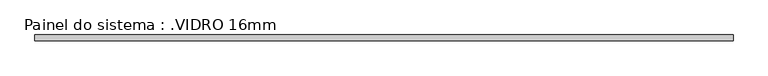
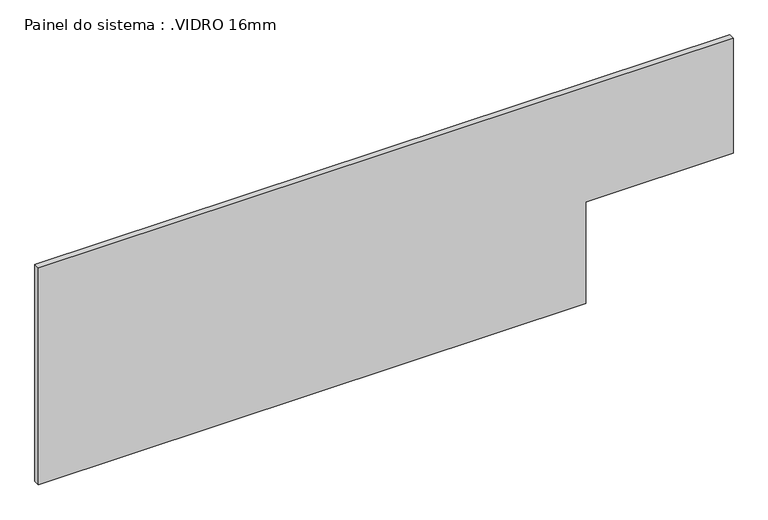
"""IFC4 building model written with IfcOpenShell, lengths in millimetres: plate geometry, Painel do sistema : .VIDRO 16mm."""

from ifc_helpers import new_model, si_unit, frame, origin, place, context, project, spatial, polyline, outline, extrude, source, transform, mapped, element, save


def painel_do_sistema_vidro_16mm_d2e68e8b(model_context):
    return source(origin(), model_context, "Body", "SweptSolid", [
        extrude(outline(polyline([(0.0, -942.5), (0.0, 542.5), (291.6666667, 542.5), (291.6666667, 942.5), (621.6666667, 942.5), (621.6666667, -942.5), (0.0, -942.5)])), frame((0.0, -200.0, 0.0), z_axis=(0.0, 1.0, 0.0), x_axis=(0.0, 0.0, 1.0)), (0.0, 0.0, 1.0), 16.0),
    ])


if __name__ == "__main__":
    model = new_model("IFC4")
    model_context = context("Model", 3, world=origin())
    ifc_project = project(units=[si_unit("LENGTHUNIT", "METRE", prefix="MILLI")], contexts=[model_context])
    site = spatial("IfcSite", under=ifc_project)
    building = spatial("IfcBuilding", under=site)
    placement = place(None, origin())
    painel_do_sistema_vidro_16mm_shape = painel_do_sistema_vidro_16mm_d2e68e8b(model_context)
    element("IfcPlate", 1, ObjectType="Painel do sistema : .VIDRO 16mm", at=placement, inside=building, context=model_context, shape_type="MappedRepresentation", body=[
        mapped(painel_do_sistema_vidro_16mm_shape, transform((0.0, 0.0, 0.0), x_axis=(1.0, 0.0, 0.0), y_axis=(0.0, 1.0, 0.0), z_axis=(0.0, 0.0, 1.0))),
    ])
    save(model, "model.ifc")

# Revit data of these elements
# Element 1 (IfcPlate, "Painel do sistema : .VIDRO 16mm")
#   Materials on its faces: ".VIDRO"
# Materials
#   ".VIDRO": class "Genérico", colour RGB 198 236 255, transparency 0.95, Cost = 0
